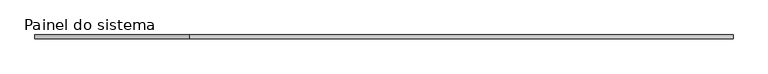
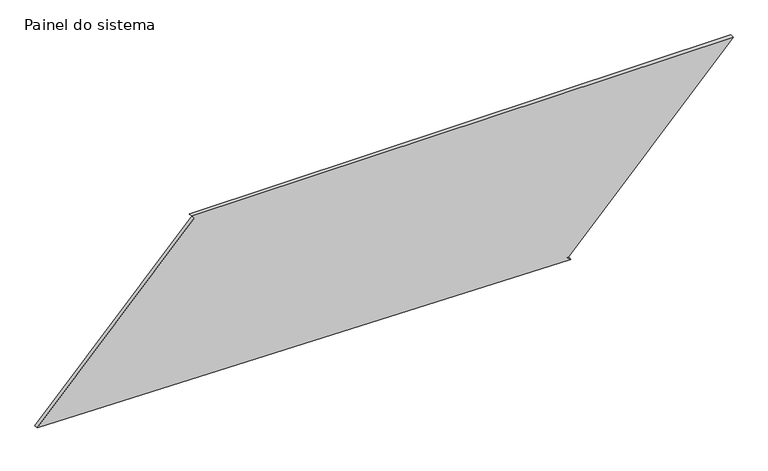
"""IFC4 building model written with IfcOpenShell, lengths in millimetres: plate geometry, Painel do sistema : Envidraçado."""

from ifc_helpers import new_model, si_unit, frame, origin, place, context, project, spatial, polyline, outline, extrude, source, transform, mapped, element, save


def painel_do_sistema_c0c56a08(model_context):
    return source(origin(), model_context, "Body", "SweptSolid", [
        extrude(outline(polyline([(0.0, 1198.7093866), (17.1196584, 1180.490789), (1151.8758999, 2246.7989467), (1151.8758999, -1249.1190705), (1134.7562416, -1230.9004729), (53.6455649, -2246.7989467), (0.0, 1198.7093866)])), frame((0.0, 24.5, 0.0), z_axis=(0.0, 1.0, 0.0), x_axis=(0.0, 0.0, 1.0)), (0.0, 0.0, 1.0), 25.0),
    ])


if __name__ == "__main__":
    model = new_model("IFC4")
    model_context = context("Model", 3, world=origin())
    ifc_project = project(units=[si_unit("LENGTHUNIT", "METRE", prefix="MILLI")], contexts=[model_context])
    site = spatial("IfcSite", under=ifc_project)
    building = spatial("IfcBuilding", under=site)
    placement = place(None, origin())
    painel_do_sistema_shape = painel_do_sistema_c0c56a08(model_context)
    element("IfcPlate", 1, ObjectType="Painel do sistema : Envidraçado", at=placement, inside=building, context=model_context, shape_type="MappedRepresentation", body=[
        mapped(painel_do_sistema_shape, transform((0.0, 0.0, 0.0), x_axis=(1.0, 0.0, 0.0), y_axis=(0.0, 1.0, 0.0), z_axis=(0.0, 0.0, 1.0))),
    ])
    save(model, "model.ifc")

# Revit data of these elements
# Type "Painel do sistema : Envidraçado"
#   Construction Type Id = "GSP4R"
#   Analytic Construction = "Vidraça única Pilkington 1/8 pol"
#   Visual Light Transmittance = 0.9
#   Solar Heat Gain Coefficient = 0.86
#   Heat Transfer Coefficient (U) = 6.7069 W/(m²·K)
# Element 1 (IfcPlate, "Painel do sistema : Envidraçado")
#   Materials on its faces: "Vidro"
# Materials
#   "Vidro": class "Vidro", colour RGB 0 128 192, transparency 0.9, Description = "Vidro de sílica", Cost = 0
